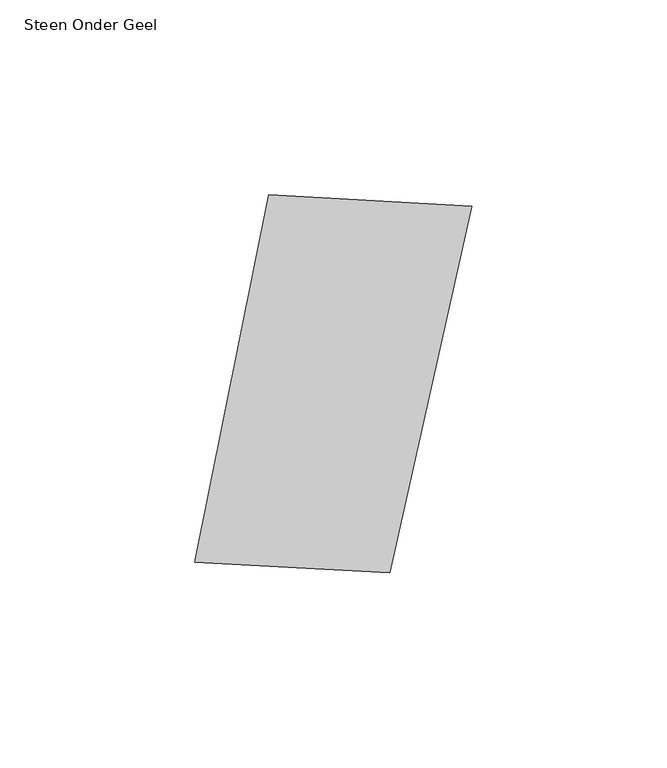
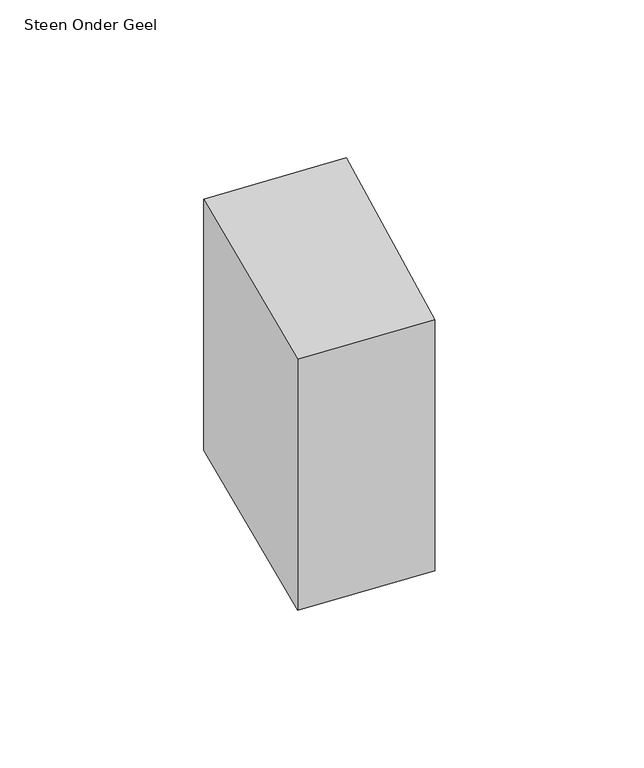
"""IFC4 building model written with IfcOpenShell, lengths in millimetres: proxy geometry, 00_GMA_steen_versie_4 : Steen Onder Geel."""

from ifc_helpers import new_model, si_unit, origin, origin_with_axes, place, context, project, spatial, polyline, outline, extrude, source, transform, mapped, element, save


def steen_onder_geel_091d2dd8(model_context):
    return source(origin(), model_context, "Body", "SweptSolid", [
        extrude(outline(polyline([(110.556194, 113.4547711), (89.4714938, 19.4113541), (39.5482131, 22.1801158), (58.5203525, 116.3266865), (110.556194, 113.4547711)])), origin_with_axes(), (0.0, 0.0, 1.0), 100.0),
    ])


if __name__ == "__main__":
    model = new_model("IFC4")
    model_context = context("Model", 3, world=origin())
    ifc_project = project(units=[si_unit("LENGTHUNIT", "METRE", prefix="MILLI")], contexts=[model_context])
    site = spatial("IfcSite", under=ifc_project)
    building = spatial("IfcBuilding", under=site)
    placement = place(None, origin())
    steen_onder_geel_shape = steen_onder_geel_091d2dd8(model_context)
    element("IfcBuildingElementProxy", 1, Name="00_GMA_steen_versie_4 : Steen Onder Geel", ObjectType="00_GMA_steen_versie_4 : Steen Onder Geel", at=placement, inside=building, context=model_context, shape_type="MappedRepresentation", body=[
        mapped(steen_onder_geel_shape, transform((0.0, 0.0, 0.0), x_axis=(1.0, 0.0, 0.0), y_axis=(0.0, 1.0, 0.0), z_axis=(0.0, 0.0, 1.0))),
    ])
    save(model, "model.ifc")

# Revit data of these elements
# Type "00_GMA_steen_versie_4 : Steen Onder Geel"
#   StootVoegHalfBoven [instance default] = 5 mm
#   StootVoegHalf [instance default] = 5 mm
#   StootVoegBreedteOnder = 10 mm
#   StootVoegBreedteBoven = 10 mm
#   Steendikte = 100 mm
#   LintVoegOnderHalf = 0 mm
#   LintVoegOnder = 0 mm
#   LintVoegBovenHalf = 5 mm
#   LintVoegBoven = 10 mm
#   materiaal = 21_steen_geel
#   MateriaalVoeg = none
#   Default Elevation = 0
# Element 1 (IfcBuildingElementProxy, "00_GMA_steen_versie_4 : Steen Onder Geel")
#   Materials on its faces: "21_steen_geel"
# Materials
#   "21_steen_geel": class "Unassigned", colour RGB 202 202 0, transparency 0, Cost = 0
